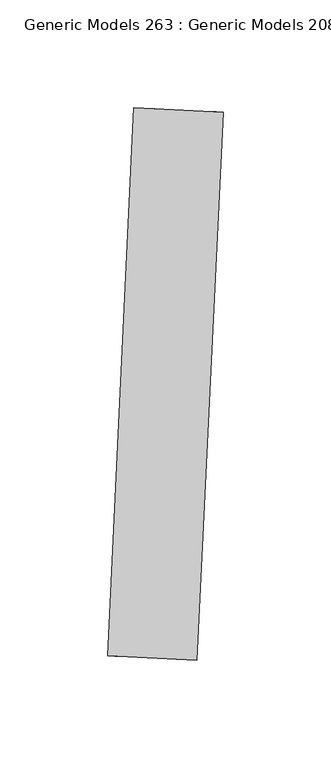
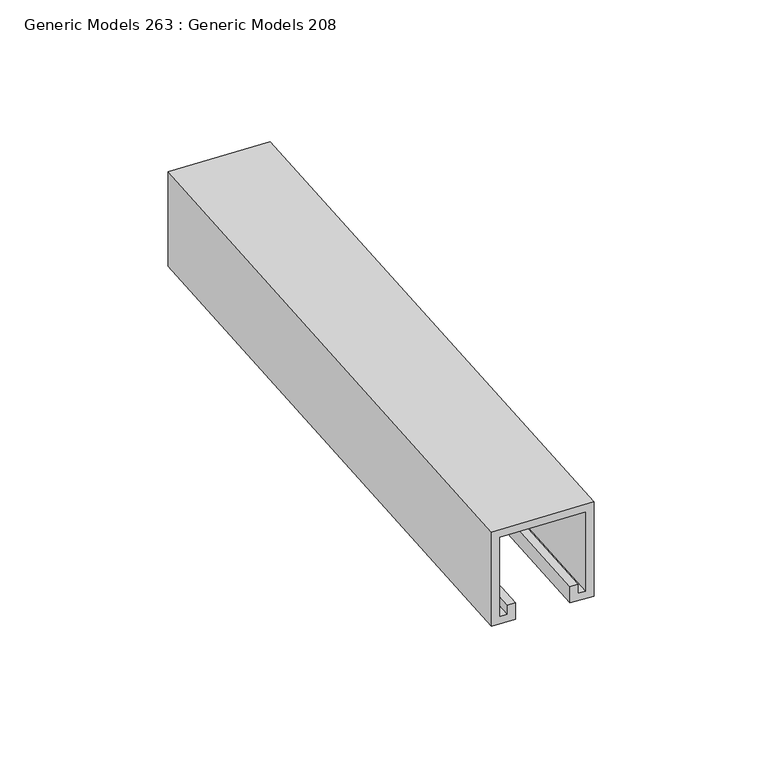
"""IFC4 building model written with IfcOpenShell, lengths in millimetres: proxy geometry, Generic Models 263 : Generic Models 208."""

import ifcopenshell
import ifcopenshell.guid

model = None  # the IFC model being written
_history = None  # IfcOwnerHistory: only IFC2X3 demands one
_inside = {}  # id of a spatial element -> (the spatial element, [elements in it])
_under = {}  # id of a project, library or spatial element -> (it, [spatial elements below it])
_declared = {}  # id of a project -> (the project, [libraries it declares])
_typed = {}  # id of a type object -> (the type object, [elements of that type])
_made_of = {}  # id of a material, layer set ... -> (it, [elements and type objects made of it])


def new_model(schema):
    """Start an empty IFC model of exactly this schema.

    Asked for "IFC4X3", IfcOpenShell would pick the latest addendum, in which some entities
    have other attributes; the version numbers below select the first issue.
    IFC2X3 requires an IfcOwnerHistory on every rooted entity: one is made here for all.
    """
    global model, _history
    if schema == "IFC4X3":
        model = ifcopenshell.file(schema_version=(4, 3, 0, 0))
    else:
        model = ifcopenshell.file(schema=schema)
    _inside.clear()
    _under.clear()
    _declared.clear()
    _typed.clear()
    _made_of.clear()
    _history = None
    if model.schema == "IFC2X3":
        org = make("IfcOrganization", Name="unknown")
        user = make(
            "IfcPersonAndOrganization",
            ThePerson=make("IfcPerson", FamilyName="unknown"),
            TheOrganization=org,
        )
        app = make(
            "IfcApplication",
            ApplicationDeveloper=org,
            Version="unknown",
            ApplicationFullName="unknown",
            ApplicationIdentifier="unknown",
        )
        _history = make(
            "IfcOwnerHistory",
            OwningUser=user,
            OwningApplication=app,
            ChangeAction="ADDED",
            CreationDate=0,
        )
    return model


def make(cls, **values):
    """One entity of the class cls with the attributes given. An attribute that is None is left unset."""
    return model.create_entity(
        cls, **{name: value for name, value in values.items() if value is not None}
    )


def rooted(cls, **values):
    """An entity with a GlobalId (a new one), such as an element, a storey or a relation."""
    return make(cls, GlobalId=ifcopenshell.guid.new(), OwnerHistory=_history, **values)


def si_unit(unit_type, name, prefix=None):
    """IfcSIUnit, for example si_unit("LENGTHUNIT", "METRE", prefix="MILLI")."""
    return make("IfcSIUnit", UnitType=unit_type, Prefix=prefix, Name=name)


def assignment(units):
    """IfcUnitAssignment: the units of a project."""
    return None if units is None else make("IfcUnitAssignment", Units=units)


def point(xyz):
    """IfcCartesianPoint."""
    return None if xyz is None else make("IfcCartesianPoint", Coordinates=xyz)


def direction(xyz):
    """IfcDirection."""
    return None if xyz is None else make("IfcDirection", DirectionRatios=xyz)


def frame(location, z_axis=None, x_axis=None):
    """IfcAxis2Placement3D, a coordinate frame: its origin and axes. An axis left out is left unset."""
    return make(
        "IfcAxis2Placement3D",
        Location=point(location),
        Axis=direction(z_axis),
        RefDirection=direction(x_axis),
    )


def origin():
    """The frame at (0, 0, 0) with its axes left unset."""
    return frame((0.0, 0.0, 0.0))


def place(relative_to, where):
    """IfcLocalPlacement: puts the frame where relative to a parent placement (None: the world)."""
    return make(
        "IfcLocalPlacement", PlacementRelTo=relative_to, RelativePlacement=where
    )


def context(
    kind, dimensions, precision=None, world=None, true_north=None, identifier=None
):
    """IfcGeometricRepresentationContext, for example the 3D "Model" context."""
    return make(
        "IfcGeometricRepresentationContext",
        ContextIdentifier=identifier,
        ContextType=kind,
        CoordinateSpaceDimension=dimensions,
        Precision=precision,
        WorldCoordinateSystem=world,
        TrueNorth=true_north,
    )


def project(units=None, contexts=None):
    """IfcProject with its units and contexts."""
    return rooted(
        "IfcProject",
        Name="project",
        RepresentationContexts=contexts,
        UnitsInContext=assignment(units),
    )


def spatial(cls, under=None, at=None, **own):
    """A site, building, storey or space (cls), placed at a placement, below another one or the project."""
    s = rooted(cls, ObjectPlacement=at, **own)
    if under is not None:
        _under.setdefault(under.id(), (under, []))[1].append(s)
    return s


def polyline(points):
    """IfcPolyline through the points."""
    return make("IfcPolyline", Points=[point(p) for p in points])


def outline(outer, holes=None, kind="AREA"):
    """IfcArbitraryClosedProfileDef: a profile drawn as a closed curve; with holes, ...WithVoids."""
    if holes is None:
        return make("IfcArbitraryClosedProfileDef", ProfileType=kind, OuterCurve=outer)
    return make(
        "IfcArbitraryProfileDefWithVoids",
        ProfileType=kind,
        OuterCurve=outer,
        InnerCurves=holes,
    )


def extrude(swept, where, along, depth):
    """IfcExtrudedAreaSolid: the profile swept, set in the frame where, extruded along a direction by depth."""
    return make(
        "IfcExtrudedAreaSolid",
        SweptArea=swept,
        Position=where,
        ExtrudedDirection=direction(along),
        Depth=depth,
    )


def shape(context_of_items, identifier, shape_type, items):
    """IfcShapeRepresentation: the items that make up one representation, for example the "Body"."""
    return make(
        "IfcShapeRepresentation",
        ContextOfItems=context_of_items,
        RepresentationIdentifier=identifier,
        RepresentationType=shape_type,
        Items=items,
    )


def source(mapping_origin, context_of_items, identifier, shape_type, items):
    """IfcRepresentationMap: a shape defined once, which mapped items show again and again."""
    return make(
        "IfcRepresentationMap",
        MappingOrigin=mapping_origin,
        MappedRepresentation=shape(context_of_items, identifier, shape_type, items),
    )


def transform(
    local_origin,
    x_axis=None,
    y_axis=None,
    z_axis=None,
    scale=None,
    scale2=None,
    scale3=None,
    uniform=True,
):
    """IfcCartesianTransformationOperator3D, or its non-uniform kind. x_axis, y_axis, z_axis: its Axis1, 2, 3."""
    if uniform:
        return make(
            "IfcCartesianTransformationOperator3D",
            Axis1=direction(x_axis),
            Axis2=direction(y_axis),
            LocalOrigin=point(local_origin),
            Scale=scale,
            Axis3=direction(z_axis),
        )
    return make(
        "IfcCartesianTransformationOperator3DnonUniform",
        Axis1=direction(x_axis),
        Axis2=direction(y_axis),
        LocalOrigin=point(local_origin),
        Scale=scale,
        Axis3=direction(z_axis),
        Scale2=scale2,
        Scale3=scale3,
    )


def mapped(mapping_source, mapping_target):
    """IfcMappedItem: shows the shape of a source again, moved by a transform."""
    return make(
        "IfcMappedItem", MappingSource=mapping_source, MappingTarget=mapping_target
    )


def made_of(thing, what):
    """Note that an element or type object is made of a material, layer set ...; save() writes the relation."""
    if what is not None:
        _made_of.setdefault(what.id(), (what, []))[1].append(thing)
    return thing


def element(
    cls,
    number,
    at=None,
    inside=None,
    cuts=None,
    type_object=None,
    material=None,
    context=None,
    identifier="Body",
    shape_type=None,
    held_by="IfcProductDefinitionShape",
    body=None,
    shapes=None,
    **own,
):
    """One element of the class cls, such as IfcWall. Its Tag is "e" and its number.

    at: its placement. inside: the storey or other place that contains it. cuts: it is an
    opening in that element (IfcRelVoidsElement). A single representation is given by context,
    identifier, shape_type and body (its items); several are given by shapes. held_by: the class
    of the entity that holds the representations. save() writes the other relations.
    """
    e = rooted(cls, Tag="e%d" % number, ObjectPlacement=at, **own)
    if body is not None:
        shapes = [shape(context, identifier, shape_type, body)]
    if shapes is not None:
        e.Representation = make(held_by, Representations=shapes)
    if inside is not None:
        _inside.setdefault(inside.id(), (inside, []))[1].append(e)
    if cuts is not None:
        rooted(
            "IfcRelVoidsElement", RelatingBuildingElement=cuts, RelatedOpeningElement=e
        )
    if type_object is not None:
        _typed.setdefault(type_object.id(), (type_object, []))[1].append(e)
    return made_of(e, material)


def aggregate(whole, parts):
    """IfcRelAggregates: a whole, such as a stair, and the parts it consists of."""
    return rooted("IfcRelAggregates", RelatingObject=whole, RelatedObjects=parts)


def save(model, path):
    """Write the relations noted so far, then the file.

    IfcRelAggregates (storeys below a building ...), IfcRelContainedInSpatialStructure (elements
    in a storey), IfcRelDefinesByType, IfcRelAssociatesMaterial and IfcRelDeclares: one each for
    every whole, place, type object, material and project.
    """
    for whole, parts in _under.values():
        aggregate(whole, parts)
    for where, things in _inside.values():
        rooted(
            "IfcRelContainedInSpatialStructure",
            RelatedElements=things,
            RelatingStructure=where,
        )
    for kind, things in _typed.values():
        rooted("IfcRelDefinesByType", RelatedObjects=things, RelatingType=kind)
    for what, things in _made_of.values():
        rooted("IfcRelAssociatesMaterial", RelatedObjects=things, RelatingMaterial=what)
    for by, libraries in _declared.values():
        rooted("IfcRelDeclares", RelatingContext=by, RelatedDefinitions=libraries)
    model.write(path)


def generic_models_263_generic_models_208_b6c354d2(model_context):
    return source(origin(), model_context, "Body", "SweptSolid", [
        extrude(outline(polyline([(-3.175, 0.0), (-3.175, 34.9250001), (-38.1, 34.9250001), (-38.1, 31.75), (-34.13125, 31.75), (-34.13125, 28.575), (-41.275, 28.575), (-41.275, 38.1000001), (0.0, 38.1000001), (0.0, -3.175), (-41.275, -3.175), (-41.275, 6.35), (-34.13125, 6.35), (-34.13125, 3.175), (-38.1, 3.175), (-38.1, 0.0), (-3.175, 0.0)])), frame((-714.913117, -22301.1148836, 1035.05), z_axis=(0.047434947939118406, 0.9988743292897326, 0.0), x_axis=(0.0, 0.0, 1.0)), (0.0, 0.0, 1.0), 254.0),
    ])


if __name__ == "__main__":
    model = new_model("IFC4")
    model_context = context("Model", 3, world=origin())
    ifc_project = project(units=[si_unit("LENGTHUNIT", "METRE", prefix="MILLI")], contexts=[model_context])
    site = spatial("IfcSite", under=ifc_project)
    building = spatial("IfcBuilding", under=site)
    placement = place(None, origin())
    generic_models_263_generic_models_208_shape = generic_models_263_generic_models_208_b6c354d2(model_context)
    element("IfcBuildingElementProxy", 1, Name="Generic Models 263 : Generic Models 208", ObjectType="Generic Models 263 : Generic Models 208", at=placement, inside=building, context=model_context, shape_type="MappedRepresentation", body=[
        mapped(generic_models_263_generic_models_208_shape, transform((0.0, 0.0, 0.0), x_axis=(1.0, 0.0, 0.0), y_axis=(0.0, 1.0, 0.0), z_axis=(0.0, 0.0, 1.0))),
    ])
    save(model, "model.ifc")

# Revit data of these elements
# Element 1 (IfcBuildingElementProxy, "Generic Models 263 : Generic Models 208")
#   Materials on its faces: "UNISTRUT P1000, 1 5/8\" X 1 5/8\", CHANNEL OR ALUM. CHANNEL"
# Materials
#   "UNISTRUT P1000, 1 5/8\" X 1 5/8\", CHANNEL OR ALUM. CHANNEL": class "Metal", colour RGB 244 244 244, transparency 0, Description = "Aluminum 6061", Cost = 0
